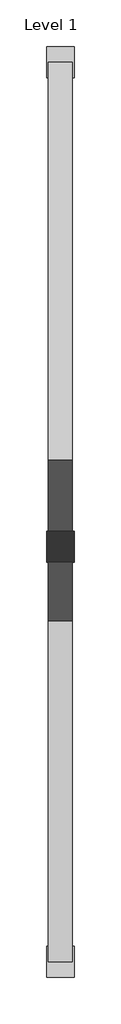
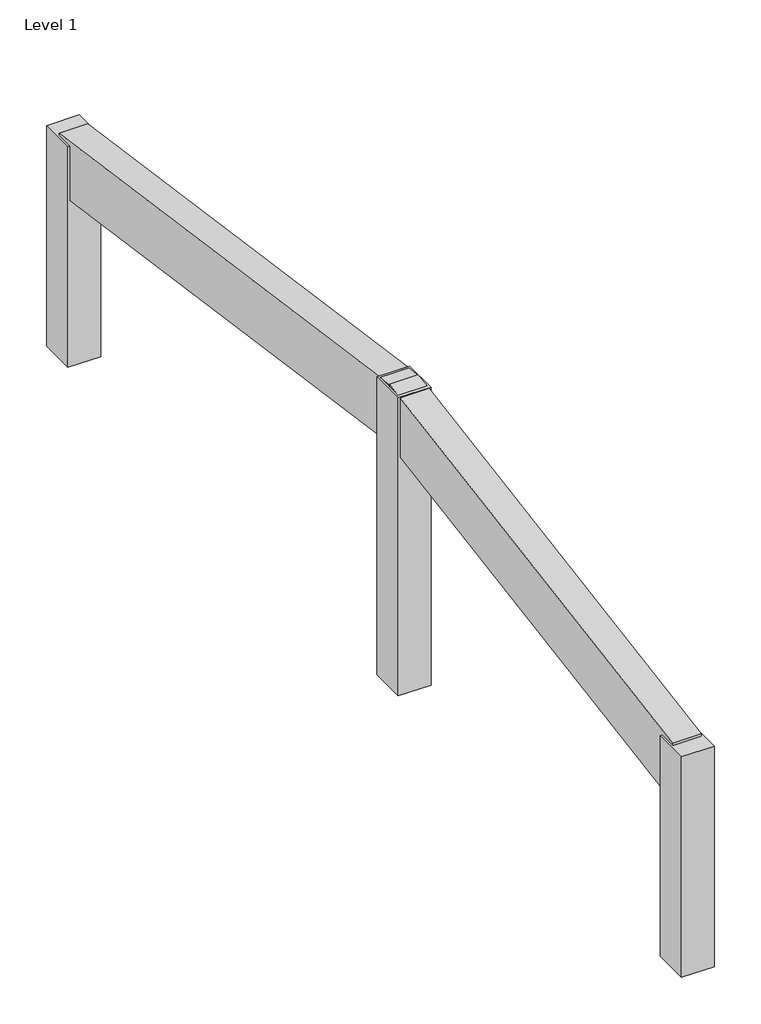
# One storey: 3 columns, 2 beams.
"""IFC4 building model written with IfcOpenShell, lengths in millimetres."""

from ifc_helpers import new_model, si_unit, frame, origin, place, context, project, spatial, polyline, outline, extrude, faceted_brep, element, save

model = new_model("IFC4")

# Units and contexts
model_context = context("Model", 3, world=origin())
ifc_project = project(units=[si_unit("LENGTHUNIT", "METRE", prefix="MILLI")], contexts=[model_context])

# Site, building, storey
site = spatial("IfcSite", under=ifc_project)
building = spatial("IfcBuilding", under=site)
storey = spatial("IfcBuildingStorey", under=building, Name="Level 1", Elevation=0.0)

# Beams
placement = place(None, origin())
element("IfcBeam", 1, ObjectType="Concrete-Rectangular Beam : 350 x 750mm 3", at=placement, inside=storey, context=model_context, shape_type="Brep", body=[
    faceted_brep([(2921.615308, 5535.5854091, 1380.1726581), (2571.615308, 5535.5854091, 1380.1726581), (2571.615308, 5354.5494602, 1350.0), (2921.615308, 5354.5494602, 1350.0), (2921.615308, 5535.5854091, 1350.0), (2921.615308, 5535.5854091, 1378.8072042), (2571.615308, 5535.5854091, 1378.8072042), (2571.615308, 5535.5854091, 1350.0)], [[[0, 1, 2, 3]], [[0, 3, 4, 5]], [[2, 1, 6, 7]], [[1, 0, 5, 4, 7, 6]], [[3, 2, 7, 4]]]),
    faceted_brep([(2921.615308, -239.4145909, -342.6726581), (2571.615308, -239.4145909, -342.6726581), (2571.615308, 5310.5854091, 582.3273419), (2921.615308, 5310.5854091, 582.3273419), (2921.615308, -464.4145909, 380.1726581), (2571.615308, -464.4145909, 380.1726581), (2571.615308, -464.4145909, 350.0), (2921.615308, -464.4145909, 350.0), (2571.615308, -239.4145909, 350.0), (2921.615308, -239.4145909, 350.0), (2571.615308, 5310.5854091, 1342.6726581), (2921.615308, 5310.5854091, 1342.6726581)], [[[0, 1, 2, 3]], [[4, 5, 6, 7]], [[8, 9, 7, 6]], [[9, 8, 1, 0]], [[10, 11, 3, 2]], [[5, 4, 11, 10]], [[4, 7, 9, 0, 3, 11]], [[6, 5, 10, 2, 1, 8]]]),
])
element("IfcBeam", 2, ObjectType="Concrete-Rectangular Beam : 350 x 750mm 3", at=placement, inside=storey, context=model_context, shape_type="SweptSolid", body=[
    extrude(outline(polyline([(12535.5854091, 350.0), (12310.5854091, 350.0), (12310.5854091, -346.6643471), (5760.5854091, 589.0499387), (5760.5854091, 1346.6643471), (12535.5854091, 378.8072042), (12535.5854091, 350.0)])), frame((2571.615308, 0.0, 0.0), z_axis=(1.0, 0.0, 0.0), x_axis=(0.0, 1.0, 0.0)), (0.0, 0.0, 1.0), 350.0),
    extrude(outline(polyline([(5535.5854091, 1378.8072042), (5737.2358385, 1350.0), (5535.5854091, 1350.0), (5535.5854091, 1378.8072042)])), frame((2571.615308, 0.0, 0.0), z_axis=(1.0, 0.0, 0.0), x_axis=(0.0, 1.0, 0.0)), (0.0, 0.0, 1.0), 350.0),
])

# Columns
element("IfcColumn", 3, ObjectType="Concrete-Rectangular-Column : 400 x 450mm 2", at=placement, inside=storey, context=model_context, shape_type="SweptSolid", body=[
    extrude(outline(polyline([(2946.615308, -239.4145909), (2946.615308, -689.4145909), (2546.615308, -689.4145909), (2546.615308, -239.4145909), (2946.615308, -239.4145909)])), frame((0.0, 0.0, -2500.0), z_axis=(0.0, 0.0, 1.0), x_axis=(1.0, 0.0, 0.0)), (0.0, 0.0, 1.0), 2850.0),
])
element("IfcColumn", 4, ObjectType="Concrete-Rectangular-Column : 400 x 450mm 2", at=placement, inside=storey, context=model_context, shape_type="SweptSolid", body=[
    extrude(outline(polyline([(2946.615308, 5760.5854091), (2946.615308, 5310.5854091), (2546.615308, 5310.5854091), (2546.615308, 5760.5854091), (2946.615308, 5760.5854091)])), frame((0.0, 0.0, -2500.0), z_axis=(0.0, 0.0, 1.0), x_axis=(1.0, 0.0, 0.0)), (0.0, 0.0, 1.0), 3850.0),
])
element("IfcColumn", 5, ObjectType="Concrete-Rectangular-Column : 400 x 450mm 2", at=placement, inside=storey, context=model_context, shape_type="Brep", body=[
    faceted_brep([(2946.615308, 12760.5854091, 350.0), (2546.615308, 12760.5854091, 350.0), (2546.615308, 12310.5854091, 350.0), (2571.615308, 12310.5854091, 350.0), (2921.615308, 12310.5854091, 350.0), (2946.615308, 12310.5854091, 350.0), (2946.615308, 12760.5854091, -2500.0), (2946.615308, 12310.5854091, -2500.0), (2546.615308, 12310.5854091, -2500.0), (2546.615308, 12760.5854091, -2500.0)], [[[0, 1, 2, 3, 4, 5]], [[6, 7, 8, 9]], [[1, 0, 6, 9]], [[2, 1, 9, 8]], [[5, 4, 3, 2, 8, 7]], [[0, 5, 7, 6]]]),
])

save(model, "model.ifc")

# Revit data of these elements
# Project information
#   Fecha de emisión de proyecto = "Issue Date"
#   Estado de proyecto = "Project Status"
#   Nombre de cliente = "Owner"
#   Dirección de proyecto = "Enter address here"
#   Nombre de proyecto = "Project Name"
#   Número de proyecto = "Project Number"
# Type "Concrete-Rectangular Beam : 350 x 750mm 3"
#   Length [instance default] = 1524 mm
#   b = 350 mm
#   h = 750 mm
#   Structural Material [instance default] = Concrete, Cast-in-Place gray
#   Assembly Code = ""
# Type "Concrete-Rectangular-Column : 400 x 450mm 2"
#   b = 400 mm
#   h = 450 mm
#   Structural Material [instance default] = Concrete, Cast-in-Place gray
# Elements 1, 2 (IfcBeam, "Concrete-Rectangular Beam : 350 x 750mm 3")
#   Structural Material = Concrete, Cast-in-Place gray
#   Phase Created = New Construction
#   Materials on its faces: "Concrete, Cast-in-Place gray"
# Elements 3, 4, 5 (IfcColumn, "Concrete-Rectangular-Column : 400 x 450mm 2")
#   Structural Material = Concrete, Cast-in-Place gray
#   Phase Created = New Construction
#   Materials on its faces: "Concrete, Cast-in-Place gray"
# Materials
#   "Concrete, Cast-in-Place gray": class "Concrete", colour RGB 192 192 192, transparency 0, Description = "Cast-in-place concrete", Cost = 0
